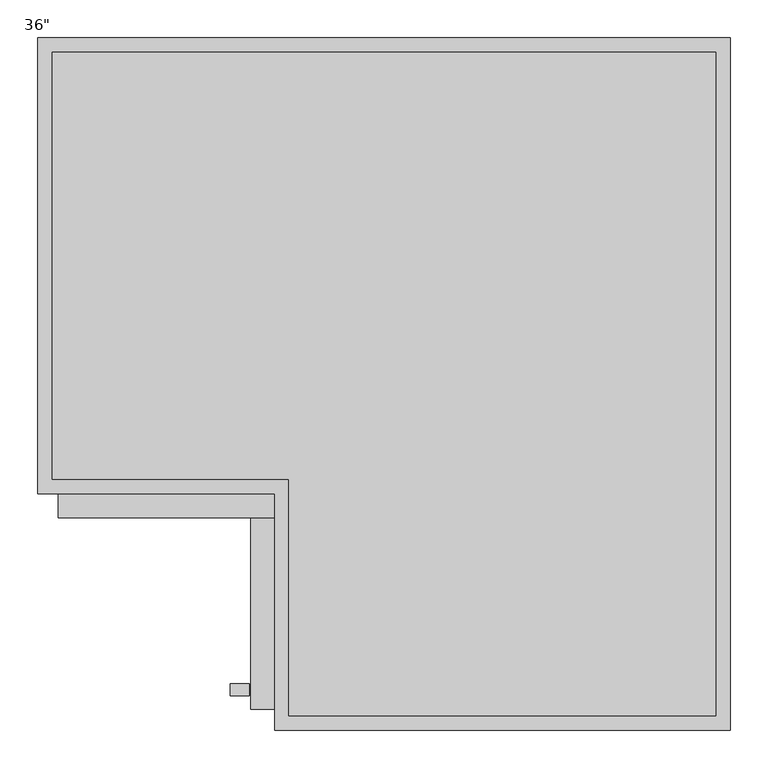
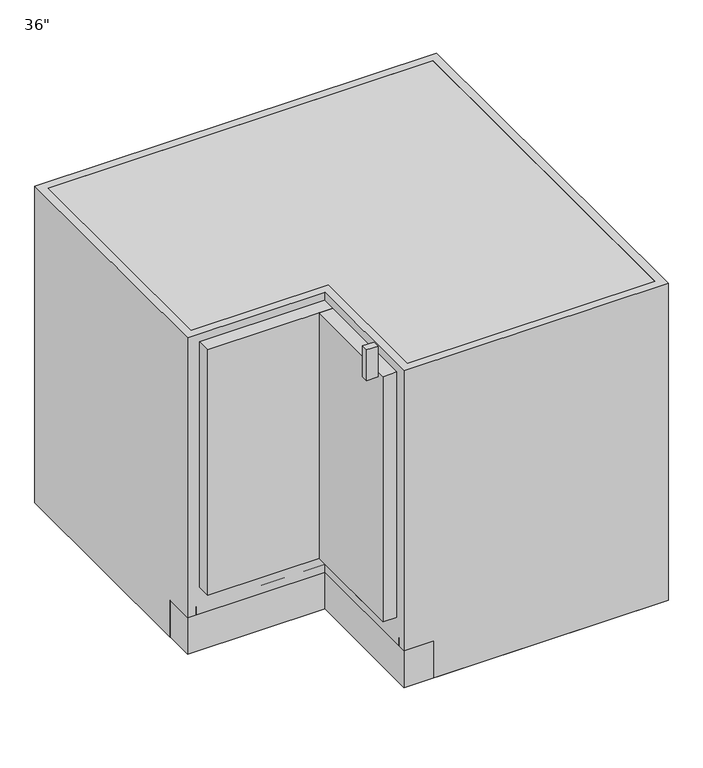
"""IFC4 building model written with IfcOpenShell, lengths in millimetres: furniture geometry."""

from ifc_helpers import new_model, si_unit, point, frame, frame_2d, origin, origin_with_axes, place, context, project, spatial, polyline, circle_curve, trimmed, segment, composite_curve, outline, extrude, faceted_brep, source, transform, mapped, element, save


def furniture_b207726a(model_context):
    return source(origin(), model_context, "Body", "SolidModel", [
        extrude(outline(polyline([(-74.9665215, -633.9456685), (-360.4850858, -634.2486655), (-360.5187794, -602.4986834), (-75.0002151, -602.1956864), (-74.9665215, -633.9456685)])), frame((0.0, 0.0, 152.4), z_axis=(0.0, 0.0, 1.0), x_axis=(1.0, 0.0, 0.0)), (0.0, 0.0, 1.0), 590.55),
        faceted_brep([(526.7377049, 0.0, 762.0), (-387.6622951, 0.0, 762.0), (-387.6622951, -602.3436184, 762.0), (-74.9833665, -602.3436184, 762.0), (-74.9833665, -914.4, 762.0), (526.7377049, -914.4, 762.0), (507.6877049, -895.35, 762.0), (-55.9333665, -895.35, 762.0), (-55.9333665, -583.2936184, 762.0), (-368.6122951, -583.2936184, 762.0), (-368.6122951, -19.05, 762.0), (507.6877049, -19.05, 762.0), (-74.9833665, -914.4, 88.9), (-74.9833665, -602.3436184, 88.9), (-387.6622951, -602.3436184, 88.9), (-387.6622951, -534.0223805, 88.9), (-368.6122951, -534.0223805, 88.9), (-368.6122951, -583.2936184, 88.9), (-55.9333665, -583.2936184, 88.9), (-55.9333665, -895.35, 88.9), (-6.6622951, -895.35, 88.9), (-6.6622951, -914.4, 88.9), (526.7377049, 0.0, 0.0), (-387.6622951, 0.0, 0.0), (-387.6622951, -534.0223805, 0.0), (-6.6622951, -914.4, 0.0), (526.7377049, -914.4, 0.0), (507.6877049, -895.35, 88.9), (-368.6122951, -19.05, 88.9), (507.6877049, -19.05, 88.9), (-6.6622951, -534.0223805, 88.9), (-6.6622951, -534.0223805, 0.0)], [[[0, 1, 2, 3, 4, 5], [6, 7, 8, 9, 10, 11]], [[12, 13, 14, 15, 16, 17, 18, 19, 20, 21]], [[1, 0, 22, 23]], [[2, 1, 23, 24, 15, 14]], [[3, 2, 14, 13]], [[4, 3, 13, 12]], [[5, 4, 12, 21, 25, 26]], [[22, 0, 5, 26]], [[7, 6, 27, 20, 19]], [[8, 7, 19, 18]], [[9, 8, 18, 17]], [[10, 9, 17, 16, 28]], [[11, 10, 28, 29]], [[6, 11, 29, 27]], [[16, 30, 20, 27, 29, 28]], [[22, 26, 25, 31, 24, 23]], [[24, 31, 30, 16, 15]], [[31, 25, 21, 20, 30]]]),
        extrude(outline(polyline([(507.6877049, -19.05), (507.6877049, -895.35), (-74.9833665, -895.35), (-74.9833665, -602.3436184), (-368.6122951, -602.3436184), (-368.6122951, -19.05), (507.6877049, -19.05)])), frame((0.0, 0.0, 88.9), z_axis=(0.0, 0.0, 1.0), x_axis=(1.0, 0.0, 0.0)), (0.0, 0.0, 1.0), 19.05),
        extrude(outline(polyline([(526.7377049, 0.0), (526.7377049, -914.4), (-74.9833665, -914.4), (-74.9833665, -602.3436184), (-387.6622951, -602.3436184), (-387.6622951, 0.0), (526.7377049, 0.0)])), origin_with_axes(), (0.0, 0.0, 1.0), 762.0),
        extrude(outline(composite_curve([segment(trimmed(circle_curve(frame_2d((85.8132868, -441.5469651)), 19.05), [point((66.7632868, -441.5469651))], [point((104.8632868, -441.5469651))], False, "CARTESIAN"), True, "CONTINUOUS"), segment(trimmed(circle_curve(frame_2d((85.8132868, -441.5469651)), 19.05), [point((104.8632868, -441.5469651))], [point((66.7632868, -441.5469651))], False, "CARTESIAN"), True, "CONTINUOUS")], self_intersect=False)), origin_with_axes(), (0.0, 0.0, 1.0), 742.95),
        extrude(outline(composite_curve([segment(trimmed(circle_curve(frame_2d((71.0113229, -457.5795168)), 423.5329098), [point((-338.2830079, -566.4752307))], [point((-36.9637809, -867.1176746))], False, "CARTESIAN"), True, "CONTINUOUS"), segment(polyline([(-36.9637809, -867.1176746), (-36.9637809, -566.4752307), (-338.2830079, -566.4752307)]), True, "CONTINUOUS")], self_intersect=False)), frame((0.0, 0.0, 203.2), z_axis=(0.0, 0.0, 1.0), x_axis=(1.0, 0.0, 0.0)), (0.0, 0.0, 1.0), 45.0692226),
        extrude(outline(polyline([(-108.2622951, -853.255371), (-108.2622951, -869.0436184), (-133.6622951, -869.0436184), (-133.6622951, -853.255371), (-108.2622951, -853.255371)])), frame((0.0, 0.0, 732.086599), z_axis=(0.0, 0.0, 1.0), x_axis=(1.0, 0.0, 0.0)), (0.0, 0.0, 1.0), 73.5640045),
        extrude(outline(polyline([(-74.9833665, -886.7884981), (-106.5244839, -886.7884981), (-106.5244839, -634.3478814), (-74.9833665, -634.3478814), (-74.9833665, -886.7884981)])), frame((0.0, 0.0, 152.4), z_axis=(0.0, 0.0, 1.0), x_axis=(1.0, 0.0, 0.0)), (0.0, 0.0, 1.0), 590.55),
    ])


if __name__ == "__main__":
    model = new_model("IFC4")
    model_context = context("Model", 3, world=origin())
    ifc_project = project(units=[si_unit("LENGTHUNIT", "METRE", prefix="MILLI")], contexts=[model_context])
    site = spatial("IfcSite", under=ifc_project)
    building = spatial("IfcBuilding", under=site)
    placement = place(None, origin())
    furniture_shape = furniture_b207726a(model_context)
    element("IfcFurniture", 1, ObjectType="36039039_Lazy_Susan_Base_Corner_Cabinet_with_ONE_rotating_shelf_14808 (1) : 36\"", at=placement, inside=building, context=model_context, shape_type="MappedRepresentation", body=[
        mapped(furniture_shape, transform((0.0, 0.0, 0.0), x_axis=(1.0, 0.0, 0.0), y_axis=(0.0, 1.0, 0.0), z_axis=(0.0, 0.0, 1.0))),
    ])
    save(model, "model.ifc")

# Revit data of these elements
# Type "36039039_Lazy_Susan_Base_Corner_Cabinet_with_ONE_rotating_shelf_14808 (1) : 36\""
#   Assembly Code = "C1030410"
#   Depth = 3' - 0"
#   Height = 2' - 6"
#   Toe Height = 0' - 3 1/2"
#   Width = 3' - 0"
#   Cabinet Material = Red Oak Low Gloss
#   Door/Drawer Material = none
#   Default Elevation = 0
# Element 1 (IfcFurniture, "36039039_Lazy_Susan_Base_Corner_Cabinet_with_ONE_rotating_shelf_14808 (1) : 36\"")
#   Materials on its faces: "Red Oak Low Gloss", "Cabinets", "Poche"
# Materials
#   "Red Oak Low Gloss": class "Generic", colour RGB 127 127 127, transparency 0, Cost = 0
#   "Cabinets": class "Miscellaneous", colour RGB 249 249 249, transparency 0
#   "Poche": class "System", colour RGB 0 0 255, transparency 0, Cost = 0
